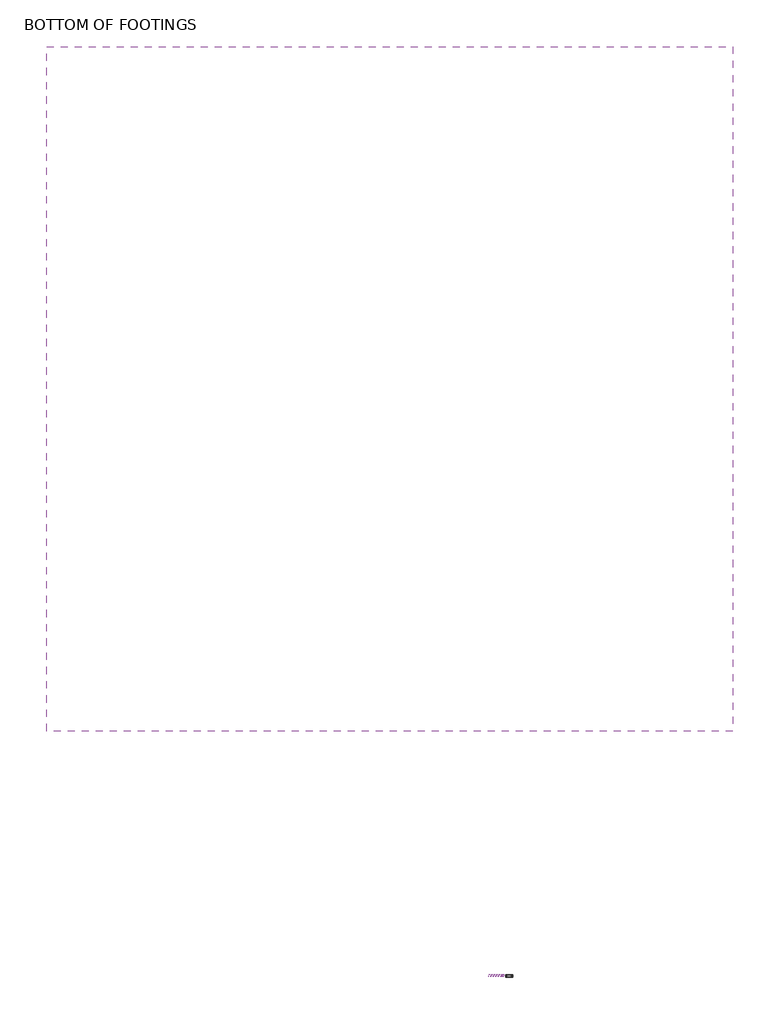
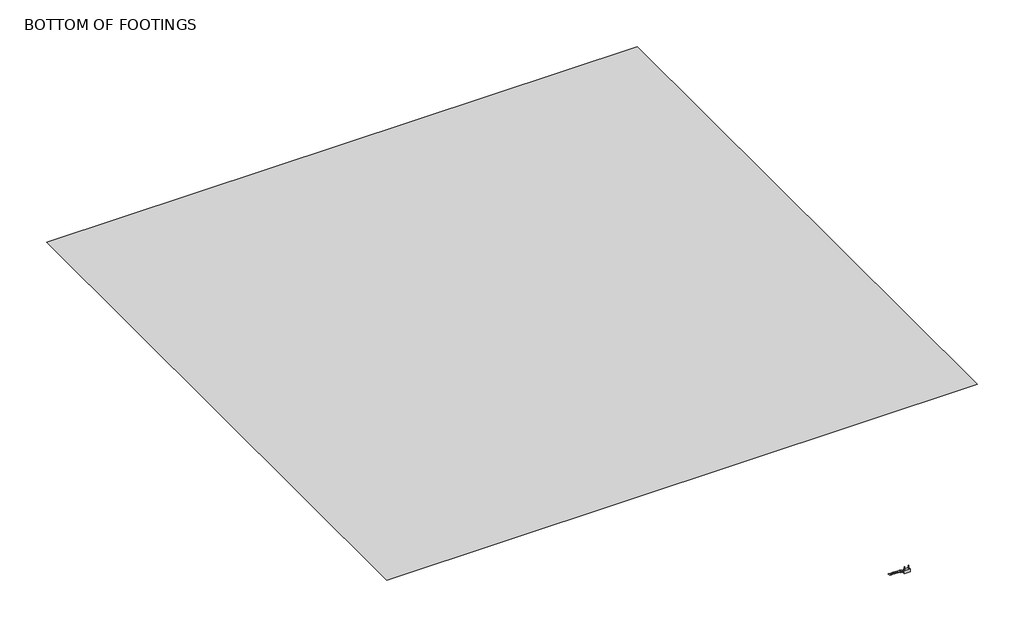
# One storey: 21 proxies.
"""IFC4 building model written with IfcOpenShell, lengths in millimetres."""

import ifcopenshell
import ifcopenshell.guid

model = None  # the IFC model being written
_history = None  # IfcOwnerHistory: only IFC2X3 demands one
_inside = {}  # id of a spatial element -> (the spatial element, [elements in it])
_under = {}  # id of a project, library or spatial element -> (it, [spatial elements below it])
_declared = {}  # id of a project -> (the project, [libraries it declares])
_typed = {}  # id of a type object -> (the type object, [elements of that type])
_made_of = {}  # id of a material, layer set ... -> (it, [elements and type objects made of it])


def new_model(schema):
    """Start an empty IFC model of exactly this schema.

    Asked for "IFC4X3", IfcOpenShell would pick the latest addendum, in which some entities
    have other attributes; the version numbers below select the first issue.
    IFC2X3 requires an IfcOwnerHistory on every rooted entity: one is made here for all.
    """
    global model, _history
    if schema == "IFC4X3":
        model = ifcopenshell.file(schema_version=(4, 3, 0, 0))
    else:
        model = ifcopenshell.file(schema=schema)
    _inside.clear()
    _under.clear()
    _declared.clear()
    _typed.clear()
    _made_of.clear()
    _history = None
    if model.schema == "IFC2X3":
        org = make("IfcOrganization", Name="unknown")
        user = make(
            "IfcPersonAndOrganization",
            ThePerson=make("IfcPerson", FamilyName="unknown"),
            TheOrganization=org,
        )
        app = make(
            "IfcApplication",
            ApplicationDeveloper=org,
            Version="unknown",
            ApplicationFullName="unknown",
            ApplicationIdentifier="unknown",
        )
        _history = make(
            "IfcOwnerHistory",
            OwningUser=user,
            OwningApplication=app,
            ChangeAction="ADDED",
            CreationDate=0,
        )
    return model


def make(cls, **values):
    """One entity of the class cls with the attributes given. An attribute that is None is left unset."""
    return model.create_entity(
        cls, **{name: value for name, value in values.items() if value is not None}
    )


def rooted(cls, **values):
    """An entity with a GlobalId (a new one), such as an element, a storey or a relation."""
    return make(cls, GlobalId=ifcopenshell.guid.new(), OwnerHistory=_history, **values)


def si_unit(unit_type, name, prefix=None):
    """IfcSIUnit, for example si_unit("LENGTHUNIT", "METRE", prefix="MILLI")."""
    return make("IfcSIUnit", UnitType=unit_type, Prefix=prefix, Name=name)


def assignment(units):
    """IfcUnitAssignment: the units of a project."""
    return None if units is None else make("IfcUnitAssignment", Units=units)


def point(xyz):
    """IfcCartesianPoint."""
    return None if xyz is None else make("IfcCartesianPoint", Coordinates=xyz)


def direction(xyz):
    """IfcDirection."""
    return None if xyz is None else make("IfcDirection", DirectionRatios=xyz)


def frame(location, z_axis=None, x_axis=None):
    """IfcAxis2Placement3D, a coordinate frame: its origin and axes. An axis left out is left unset."""
    return make(
        "IfcAxis2Placement3D",
        Location=point(location),
        Axis=direction(z_axis),
        RefDirection=direction(x_axis),
    )


def frame_2d(location, x_axis=None):
    """IfcAxis2Placement2D, a coordinate frame in the plane: its origin and x axis."""
    return make(
        "IfcAxis2Placement2D", Location=point(location), RefDirection=direction(x_axis)
    )


def origin():
    """The frame at (0, 0, 0) with its axes left unset."""
    return frame((0.0, 0.0, 0.0))


def place(relative_to, where):
    """IfcLocalPlacement: puts the frame where relative to a parent placement (None: the world)."""
    return make(
        "IfcLocalPlacement", PlacementRelTo=relative_to, RelativePlacement=where
    )


def context(
    kind, dimensions, precision=None, world=None, true_north=None, identifier=None
):
    """IfcGeometricRepresentationContext, for example the 3D "Model" context."""
    return make(
        "IfcGeometricRepresentationContext",
        ContextIdentifier=identifier,
        ContextType=kind,
        CoordinateSpaceDimension=dimensions,
        Precision=precision,
        WorldCoordinateSystem=world,
        TrueNorth=true_north,
    )


def project(units=None, contexts=None):
    """IfcProject with its units and contexts."""
    return rooted(
        "IfcProject",
        Name="project",
        RepresentationContexts=contexts,
        UnitsInContext=assignment(units),
    )


def spatial(cls, under=None, at=None, **own):
    """A site, building, storey or space (cls), placed at a placement, below another one or the project."""
    s = rooted(cls, ObjectPlacement=at, **own)
    if under is not None:
        _under.setdefault(under.id(), (under, []))[1].append(s)
    return s


def polyline(points):
    """IfcPolyline through the points."""
    return make("IfcPolyline", Points=[point(p) for p in points])


def point_list(points):
    """IfcCartesianPointList2D or 3D."""
    cls = (
        "IfcCartesianPointList2D" if len(points[0]) == 2 else "IfcCartesianPointList3D"
    )
    return make(cls, CoordList=points)


def circle_curve(where, radius):
    """IfcCircle in the frame where."""
    return make("IfcCircle", Position=where, Radius=radius)


def trimmed(basis, trim1, trim2, sense, master):
    """IfcTrimmedCurve: the piece of a basis curve between two trims."""
    return make(
        "IfcTrimmedCurve",
        BasisCurve=basis,
        Trim1=trim1,
        Trim2=trim2,
        SenseAgreement=sense,
        MasterRepresentation=master,
    )


def segment(curve, same_sense, transition):
    """IfcCompositeCurveSegment."""
    return make(
        "IfcCompositeCurveSegment",
        Transition=transition,
        SameSense=same_sense,
        ParentCurve=curve,
    )


def composite_curve(segments, self_intersect=None):
    """IfcCompositeCurve: segments joined end to end."""
    return make("IfcCompositeCurve", Segments=segments, SelfIntersect=self_intersect)


def outline(outer, holes=None, kind="AREA"):
    """IfcArbitraryClosedProfileDef: a profile drawn as a closed curve; with holes, ...WithVoids."""
    if holes is None:
        return make("IfcArbitraryClosedProfileDef", ProfileType=kind, OuterCurve=outer)
    return make(
        "IfcArbitraryProfileDefWithVoids",
        ProfileType=kind,
        OuterCurve=outer,
        InnerCurves=holes,
    )


def extrude(swept, where, along, depth):
    """IfcExtrudedAreaSolid: the profile swept, set in the frame where, extruded along a direction by depth."""
    return make(
        "IfcExtrudedAreaSolid",
        SweptArea=swept,
        Position=where,
        ExtrudedDirection=direction(along),
        Depth=depth,
    )


def faces_of(points, faces, orient=None, outer=None):
    """IfcFace entities. A face is a list of loops; a loop is a list of indices into points, from 0.

    orient and outer hold one flag for each loop. By default every Orientation is true, the
    first loop of a face is its IfcFaceOuterBound and the others are IfcFaceBound.
    """
    made = []
    for i, loops in enumerate(faces):
        bounds = []
        for j, loop in enumerate(loops):
            is_outer = j == 0 if outer is None else outer[i][j]
            bounds.append(
                make(
                    "IfcFaceOuterBound" if is_outer else "IfcFaceBound",
                    Bound=make("IfcPolyLoop", Polygon=[points[k] for k in loop]),
                    Orientation=True if orient is None else orient[i][j],
                )
            )
        made.append(make("IfcFace", Bounds=bounds))
    return made


def faceted_brep(points, faces, orient=None, outer=None, voids=None):
    """IfcFacetedBrep: a solid bounded by flat faces; with voids (closed shells), ...WithVoids."""
    shared = [point(p) for p in points]
    hull = make("IfcClosedShell", CfsFaces=faces_of(shared, faces, orient, outer))
    if voids is None:
        return make("IfcFacetedBrep", Outer=hull)
    return make(
        "IfcFacetedBrepWithVoids",
        Outer=hull,
        Voids=[
            make(cls, CfsFaces=faces_of(shared, fs, o, b)) for cls, fs, o, b in voids
        ],
    )


def triangles(points, corners, closed=None, point_numbers=None):
    """IfcTriangulatedFaceSet: each triangle names its three corners, points numbered from 1."""
    return make(
        "IfcTriangulatedFaceSet",
        Coordinates=point_list(points),
        Closed=closed,
        CoordIndex=corners,
        PnIndex=point_numbers,
    )


def shape(context_of_items, identifier, shape_type, items):
    """IfcShapeRepresentation: the items that make up one representation, for example the "Body"."""
    return make(
        "IfcShapeRepresentation",
        ContextOfItems=context_of_items,
        RepresentationIdentifier=identifier,
        RepresentationType=shape_type,
        Items=items,
    )


def source(mapping_origin, context_of_items, identifier, shape_type, items):
    """IfcRepresentationMap: a shape defined once, which mapped items show again and again."""
    return make(
        "IfcRepresentationMap",
        MappingOrigin=mapping_origin,
        MappedRepresentation=shape(context_of_items, identifier, shape_type, items),
    )


def transform(
    local_origin,
    x_axis=None,
    y_axis=None,
    z_axis=None,
    scale=None,
    scale2=None,
    scale3=None,
    uniform=True,
):
    """IfcCartesianTransformationOperator3D, or its non-uniform kind. x_axis, y_axis, z_axis: its Axis1, 2, 3."""
    if uniform:
        return make(
            "IfcCartesianTransformationOperator3D",
            Axis1=direction(x_axis),
            Axis2=direction(y_axis),
            LocalOrigin=point(local_origin),
            Scale=scale,
            Axis3=direction(z_axis),
        )
    return make(
        "IfcCartesianTransformationOperator3DnonUniform",
        Axis1=direction(x_axis),
        Axis2=direction(y_axis),
        LocalOrigin=point(local_origin),
        Scale=scale,
        Axis3=direction(z_axis),
        Scale2=scale2,
        Scale3=scale3,
    )


def mapped(mapping_source, mapping_target):
    """IfcMappedItem: shows the shape of a source again, moved by a transform."""
    return make(
        "IfcMappedItem", MappingSource=mapping_source, MappingTarget=mapping_target
    )


def made_of(thing, what):
    """Note that an element or type object is made of a material, layer set ...; save() writes the relation."""
    if what is not None:
        _made_of.setdefault(what.id(), (what, []))[1].append(thing)
    return thing


def element(
    cls,
    number,
    at=None,
    inside=None,
    cuts=None,
    type_object=None,
    material=None,
    context=None,
    identifier="Body",
    shape_type=None,
    held_by="IfcProductDefinitionShape",
    body=None,
    shapes=None,
    **own,
):
    """One element of the class cls, such as IfcWall. Its Tag is "e" and its number.

    at: its placement. inside: the storey or other place that contains it. cuts: it is an
    opening in that element (IfcRelVoidsElement). A single representation is given by context,
    identifier, shape_type and body (its items); several are given by shapes. held_by: the class
    of the entity that holds the representations. save() writes the other relations.
    """
    e = rooted(cls, Tag="e%d" % number, ObjectPlacement=at, **own)
    if body is not None:
        shapes = [shape(context, identifier, shape_type, body)]
    if shapes is not None:
        e.Representation = make(held_by, Representations=shapes)
    if inside is not None:
        _inside.setdefault(inside.id(), (inside, []))[1].append(e)
    if cuts is not None:
        rooted(
            "IfcRelVoidsElement", RelatingBuildingElement=cuts, RelatedOpeningElement=e
        )
    if type_object is not None:
        _typed.setdefault(type_object.id(), (type_object, []))[1].append(e)
    return made_of(e, material)


def aggregate(whole, parts):
    """IfcRelAggregates: a whole, such as a stair, and the parts it consists of."""
    return rooted("IfcRelAggregates", RelatingObject=whole, RelatedObjects=parts)


def save(model, path):
    """Write the relations noted so far, then the file.

    IfcRelAggregates (storeys below a building ...), IfcRelContainedInSpatialStructure (elements
    in a storey), IfcRelDefinesByType, IfcRelAssociatesMaterial and IfcRelDeclares: one each for
    every whole, place, type object, material and project.
    """
    for whole, parts in _under.values():
        aggregate(whole, parts)
    for where, things in _inside.values():
        rooted(
            "IfcRelContainedInSpatialStructure",
            RelatedElements=things,
            RelatingStructure=where,
        )
    for kind, things in _typed.values():
        rooted("IfcRelDefinesByType", RelatedObjects=things, RelatingType=kind)
    for what, things in _made_of.values():
        rooted("IfcRelAssociatesMaterial", RelatedObjects=things, RelatingMaterial=what)
    for by, libraries in _declared.values():
        rooted("IfcRelDeclares", RelatingContext=by, RelatedDefinitions=libraries)
    model.write(path)


def plane_surface(at):
    """IfcPlane: the flat surface through the origin of the frame at, square to its z axis."""
    return make("IfcPlane", Position=at)


def revolved_surface(curve, axis_point, axis_direction):
    """IfcSurfaceOfRevolution: the curve turned about the line through axis_point along axis_direction."""
    return make(
        "IfcSurfaceOfRevolution",
        SweptCurve=make("IfcArbitraryOpenProfileDef", ProfileType="CURVE", Curve=curve),
        AxisPosition=make("IfcAxis1Placement", Location=point(axis_point), Axis=direction(axis_direction)),
    )


def advanced_brep(points, edges, surfaces, faces):
    """IfcAdvancedBrep: a solid bounded by faces that lie on surfaces and meet in shared edges.

    An edge is (start, end): straight between two places in points (the first is 0);
    or (start, end, curve); or (start, end, curve, False) where it runs against its curve.
    A face is (place in surfaces, loops), or (place, loops, False) where it looks against
    its surface's normal. A loop lists edges by number (the first is 1), with a minus sign
    where the edge is run from its end to its start. The first loop is the outer one.
    """
    corners = [point(p) for p in points]
    vertices = [make("IfcVertexPoint", VertexGeometry=c) for c in corners]
    made = []
    for start, end, *more in edges:
        made.append(
            make(
                "IfcEdgeCurve",
                EdgeStart=vertices[start],
                EdgeEnd=vertices[end],
                EdgeGeometry=more[0] if more else make("IfcPolyline", Points=[corners[start], corners[end]]),
                SameSense=more[1] if len(more) > 1 else True,
            )
        )
    hull = []
    for where, loops, *sense in faces:
        bounds = []
        for j, loop in enumerate(loops):
            ring = [make("IfcOrientedEdge", EdgeElement=made[abs(k) - 1], Orientation=k > 0) for k in loop]
            bounds.append(
                make(
                    "IfcFaceOuterBound" if j == 0 else "IfcFaceBound",
                    Bound=make("IfcEdgeLoop", EdgeList=ring),
                    Orientation=True,
                )
            )
        hull.append(make("IfcAdvancedFace", Bounds=bounds, FaceSurface=surfaces[where], SameSense=sense[0] if sense else True))
    return make("IfcAdvancedBrep", Outer=make("IfcClosedShell", CfsFaces=hull))


def generic_models_129_generic_models_1_8999e842(model_context):
    return source(origin(), model_context, "Body", "SweptSolid", [
        extrude(outline(polyline([(47499.4360531, 0.0), (46280.2360531, 0.0), (46280.2360531, 1219.2), (47499.4360531, 1219.2), (47499.4360531, 0.0)])), frame((0.0, 0.0, -378.376067), z_axis=(0.0, 0.0, 1.0), x_axis=(1.0, 0.0, 0.0)), (0.0, 0.0, 1.0), 152.4),
    ])


def generic_models_131_generic_models_1_dfd9233a(model_context):
    return source(origin(), model_context, "Body", "SweptSolid", [
        extrude(outline(polyline([(-223.594817, 46885.2894531), (-224.388567, 46885.2894531), (-224.388567, 46887.8393167), (-275.188567, 46889.4367058), (-275.188567, 46890.2354003), (-224.388567, 46891.8327895), (-224.388567, 46894.3826531), (-223.594817, 46894.3826531), (-223.594817, 46885.2894531)])), frame((0.0, 565.15, 0.0), z_axis=(0.0, 1.0, 0.0), x_axis=(0.0, 0.0, 1.0)), (0.0, 0.0, 1.0), 12.7),
    ])


def generic_models_139_generic_models_1_e596f594(model_context):
    return source(origin(), model_context, "Body", "SweptSolid", [
        extrude(outline(composite_curve([segment(trimmed(circle_curve(frame_2d((97.5288266, 52112.9548165)), 6.35), [point((91.1788266, 52112.9548165))], [point((103.8788266, 52112.9548165))], False, "CARTESIAN"), True, "CONTINUOUS"), segment(trimmed(circle_curve(frame_2d((97.5288266, 52112.9548165)), 6.35), [point((103.8788266, 52112.9548165))], [point((91.1788266, 52112.9548165))], False, "CARTESIAN"), True, "CONTINUOUS")], self_intersect=False)), frame((0.0, 0.0, 0.0), z_axis=(0.0, 1.0, 0.0), x_axis=(0.0, 0.0, 1.0)), (0.0, 0.0, 1.0), 1219.2),
    ])


def generic_models_141_generic_models_1_a1e14504(model_context):
    return source(origin(), model_context, "Body", "SweptSolid", [
        extrude(outline(composite_curve([segment(trimmed(circle_curve(frame_2d((-554.7288266, 52112.9548165)), 6.35), [point((-548.3788266, 52112.9548165))], [point((-561.0788266, 52112.9548165))], False, "CARTESIAN"), True, "CONTINUOUS"), segment(trimmed(circle_curve(frame_2d((-554.7288266, 52112.9548165)), 6.35), [point((-561.0788266, 52112.9548165))], [point((-548.3788266, 52112.9548165))], False, "CARTESIAN"), True, "CONTINUOUS")], self_intersect=False)), frame((0.0, 0.0, 0.0), z_axis=(0.0, 1.0, 0.0), x_axis=(0.0, 0.0, 1.0)), (0.0, 0.0, 1.0), 1219.2),
    ])


def generic_models_144_generic_models_1_4ebe4832(model_context):
    return source(origin(), model_context, "Body", "SweptSolid", [
        extrude(outline(polyline([(-79.375, 52785.9625), (-73.025, 52785.9625), (-73.025, 52209.6280698), (-272.1843039, 52010.4687659), (-276.674432, 52014.9588939), (-79.375, 52212.2583259), (-79.375, 52785.9625)])), frame((0.0, 0.0, 0.0), z_axis=(0.0, 1.0, 0.0), x_axis=(0.0, 0.0, 1.0)), (0.0, 0.0, 1.0), 1219.2),
    ])


def generic_models_145_generic_models_1_d1ee8326(model_context):
    return source(origin(), model_context, "Body", "SweptSolid", [
        extrude(outline(polyline([(-155.575, 52785.9625), (-153.9875, 52785.9625), (-153.9875, 52482.353125), (-458.7875, 52177.553125), (-458.7875, 51873.410689), (-460.375, 51873.410689), (-460.375, 52178.210689), (-155.575, 52483.010689), (-155.575, 52785.9625)])), frame((0.0, 0.0, 0.0), z_axis=(0.0, 1.0, 0.0), x_axis=(0.0, 0.0, 1.0)), (0.0, 0.0, 1.0), 1219.2),
    ])


def generic_models_150_generic_models_1_b2c8ea2b(model_context):
    return source(origin(), model_context, "Body", "SweptSolid", [
        extrude(outline(polyline([(-310.1710164, 52787.3395874), (-157.7710164, 52787.3395874), (-157.7710164, 52483.7302124), (-462.5710164, 52178.9302124), (-462.5710164, 51824.8420742), (-513.3710164, 51824.8420742), (-513.3710164, 52343.6563593), (-310.1710164, 52546.8563593), (-310.1710164, 52787.3395874)])), frame((0.0, 0.0, 0.0), z_axis=(0.0, 1.0, 0.0), x_axis=(0.0, 0.0, 1.0)), (0.0, 0.0, 1.0), 1219.2),
    ])


def generic_models_151_generic_models_1_08f1ca75(model_context):
    return source(origin(), model_context, "Body", "SweptSolid", [
        extrude(outline(polyline([(-76.2, 51566.7625), (-685.8, 51566.7625), (-685.8, 52787.3395874), (-310.1710164, 52787.3395874), (-310.1710164, 52546.8563593), (-513.3710164, 52343.6563593), (-513.3710164, 51824.8420742), (-462.5710164, 51824.8420742), (-462.5710164, 51871.5625), (-47.9216734, 51871.5625), (-76.2, 51566.7625)])), frame((0.0, 0.0, 0.0), z_axis=(0.0, 1.0, 0.0), x_axis=(0.0, 0.0, 1.0)), (0.0, 0.0, 1.0), 1219.2),
    ])


def generic_models_177_generic_models_1_1d143019(model_context):
    return source(origin(), model_context, "Body", "Brep", [
        faceted_brep([(56665.8125, 528.6375, -1066.8), (56526.1125, 528.6375, -1066.8), (56526.1125, 528.6375, 1809.75), (56665.8125, 528.6375, 1809.75), (56665.8125, 388.9375, -1066.8), (56665.8125, 388.9375, 1809.75), (56526.1125, 388.9375, 1809.75), (56526.1125, 388.9375, -1066.8), (56545.1625, 407.9875, 1828.8), (56646.7625, 407.9875, 1828.8), (56646.7625, 509.5875, 1828.8), (56545.1625, 509.5875, 1828.8)], [[[0, 1, 2, 3]], [[4, 5, 6, 7]], [[1, 0, 4, 7]], [[2, 1, 7, 6]], [[8, 9, 10, 11]], [[0, 3, 5, 4]], [[2, 6, 8, 11]], [[5, 3, 10, 9]], [[6, 5, 9, 8]], [[3, 2, 11, 10]]]),
    ])


def generic_models_178_generic_models_155_a54ccf4c(model_context):
    return source(origin(), model_context, "Body", "SweptSolid", [
        extrude(outline(composite_curve([segment(trimmed(circle_curve(frame_2d((56595.9625, 458.7875)), 152.4), [point((56443.5625, 458.7875))], [point((56748.3625, 458.7875))], False, "CARTESIAN"), True, "CONTINUOUS"), segment(trimmed(circle_curve(frame_2d((56595.9625, 458.7875)), 152.4), [point((56748.3625, 458.7875))], [point((56443.5625, 458.7875))], False, "CARTESIAN"), True, "CONTINUOUS")], self_intersect=False)), frame((0.0, 0.0, -1219.2), z_axis=(0.0, 0.0, 1.0), x_axis=(1.0, 0.0, 0.0)), (0.0, 0.0, 1.0), 1219.2),
        extrude(outline(composite_curve([segment(trimmed(circle_curve(frame_2d((54157.5625, 458.7875)), 152.4), [point((54005.1625, 458.7875))], [point((54309.9625, 458.7875))], False, "CARTESIAN"), True, "CONTINUOUS"), segment(trimmed(circle_curve(frame_2d((54157.5625, 458.7875)), 152.4), [point((54309.9625, 458.7875))], [point((54005.1625, 458.7875))], False, "CARTESIAN"), True, "CONTINUOUS")], self_intersect=False)), frame((0.0, 0.0, -1219.2), z_axis=(0.0, 0.0, 1.0), x_axis=(1.0, 0.0, 0.0)), (0.0, 0.0, 1.0), 1219.2),
    ])


def generic_models_183_generic_models_1_4255d89c(model_context):
    return source(origin(), model_context, "Body", "Brep", [
        faceted_brep([(54227.4125, 528.6375, -1066.8), (54087.7125, 528.6375, -1066.8), (54087.7125, 528.6375, 1809.75), (54227.4125, 528.6375, 1809.75), (54227.4125, 388.9375, -1066.8), (54227.4125, 388.9375, 1809.75), (54087.7125, 388.9375, 1809.75), (54087.7125, 388.9375, -1066.8), (54106.7625, 407.9875, 1828.8), (54208.3625, 407.9875, 1828.8), (54208.3625, 509.5875, 1828.8), (54106.7625, 509.5875, 1828.8)], [[[0, 1, 2, 3]], [[4, 5, 6, 7]], [[1, 0, 4, 7]], [[2, 1, 7, 6]], [[8, 9, 10, 11]], [[0, 3, 5, 4]], [[2, 6, 8, 11]], [[5, 3, 10, 9]], [[6, 5, 9, 8]], [[3, 2, 11, 10]]]),
    ])


def generic_models_184_generic_models_184_067f22a4(model_context):
    return source(origin(), model_context, "Body", "AdvancedBrep", [
        advanced_brep(
        [(57021.4125, 977.9, -23.9117188), (53732.1125, 977.9, -23.9117188), (53732.1125, -241.3, -23.9117188), (57021.4125, -241.3, -23.9117188), (56443.5625, 458.7875, -23.9117188), (56748.3625, 458.7875, -23.9117188), (54005.1625, 458.7875, -23.9117188), (54309.9625, 458.7875, -23.9117188), (57021.4125, 977.9, -1915.3720904), (57021.4125, -241.3, -1915.3720904), (53732.1125, -241.3, -1915.3720904), (53732.1125, 977.9, -1915.3720904), (56443.5625, 458.7875, -1219.2), (56748.3625, 458.7875, -1219.2), (54005.1625, 458.7875, -1219.2), (54309.9625, 458.7875, -1219.2)],
        [
            (0, 1),
            (1, 2),
            (2, 3),
            (3, 0),
            (4, 5, circle_curve(frame((56595.9625, 458.7875, -23.9117188), z_axis=(0.0, 0.0, -1.0), x_axis=(1.0, 0.0, 0.0)), 152.4)),
            (5, 4, circle_curve(frame((56595.9625, 458.7875, -23.9117188), z_axis=(0.0, 0.0, -1.0), x_axis=(1.0, 0.0, 0.0)), 152.4)),
            (6, 7, circle_curve(frame((54157.5625, 458.7875, -23.9117188), z_axis=(0.0, 0.0, -1.0), x_axis=(1.0, 0.0, 0.0)), 152.4)),
            (7, 6, circle_curve(frame((54157.5625, 458.7875, -23.9117188), z_axis=(0.0, 0.0, -1.0), x_axis=(1.0, 0.0, 0.0)), 152.4)),
            (8, 9),
            (9, 10),
            (10, 11),
            (11, 8),
            (0, 8),
            (11, 1),
            (10, 2),
            (9, 3),
            (12, 13, circle_curve(frame((56595.9625, 458.7875, -1219.2), z_axis=(0.0, 0.0, 1.0), x_axis=(1.0, 0.0, 0.0)), 152.4)),
            (13, 12, circle_curve(frame((56595.9625, 458.7875, -1219.2), z_axis=(0.0, 0.0, 1.0), x_axis=(1.0, 0.0, 0.0)), 152.4)),
            (14, 15, circle_curve(frame((54157.5625, 458.7875, -1219.2), z_axis=(0.0, 0.0, 1.0), x_axis=(1.0, 0.0, 0.0)), 152.4)),
            (15, 14, circle_curve(frame((54157.5625, 458.7875, -1219.2), z_axis=(0.0, 0.0, 1.0), x_axis=(1.0, 0.0, 0.0)), 152.4)),
            (13, 5),
            (4, 12),
            (15, 7),
            (6, 14),
        ],
        [
            plane_surface(frame((53732.1125, 977.9, -23.9117188), z_axis=(0.0, 0.0, 1.0), x_axis=(-1.0, 0.0, 0.0))),
            plane_surface(frame((53732.1125, 977.9, -1915.3720904), z_axis=(0.0, 0.0, -1.0), x_axis=(1.0, 0.0, 0.0))),
            plane_surface(frame((57021.4125, 977.9, -23.9117188), z_axis=(0.0, 1.0, 0.0), x_axis=(0.0, 0.0, -1.0))),
            plane_surface(frame((53732.1125, 977.9, -23.9117188), z_axis=(-1.0, 0.0, 0.0), x_axis=(0.0, 0.0, -1.0))),
            plane_surface(frame((53732.1125, -241.3, -23.9117188), z_axis=(0.0, -1.0, 0.0), x_axis=(0.0, 0.0, -1.0))),
            plane_surface(frame((57021.4125, -241.3, -23.9117188), z_axis=(1.0, 0.0, 0.0), x_axis=(0.0, 0.0, -1.0))),
            plane_surface(frame((56748.3625, 458.7875, -1219.2), z_axis=(0.0, 0.0, 1.0), x_axis=(0.0, -1.0, 0.0))),
            revolved_surface(polyline([(56748.3625, 458.7875, -23.911718800000017), (56748.3625, 458.7875, -1219.2)]), (56595.9625, 458.7875, -1219.2), (0.0, 0.0, 1.0)),
            revolved_surface(polyline([(54309.9625, 458.7875, -23.9117188), (54309.9625, 458.7875, -1219.2)]), (54157.5625, 458.7875, 0.0), (0.0, 0.0, 1.0)),
        ],
        [
            (0, [[1, 2, 3, 4], [5, 6], [7, 8]]),
            (1, [[9, 10, 11, 12]]),
            (2, [[-1, 13, -12, 14]]),
            (3, [[-2, -14, -11, 15]]),
            (4, [[-3, -15, -10, 16]]),
            (5, [[-4, -16, -9, -13]]),
            (6, [[17, 18]]),
            (6, [[19, 20]]),
            (7, [[-18, 21, -5, 22]]),
            (7, [[-17, -22, -6, -21]]),
            (8, [[-20, 23, -7, 24]]),
            (8, [[-19, -24, -8, -23]]),
        ],
    ),
    ])


def generic_models_11_generic_models_1_850b304e(model_context):
    return source(origin(), model_context, "Body", "SweptSolid", [
        extrude(outline(polyline([(50347.5625, 0.0), (49128.3625, 0.0), (49128.3625, 1219.2), (50347.5625, 1219.2), (50347.5625, 0.0)])), frame((0.0, 0.0, -152.4), z_axis=(0.0, 0.0, 1.0), x_axis=(1.0, 0.0, 0.0)), (0.0, 0.0, 1.0), 152.4),
    ])


def generic_models_201_generic_models_1_6cd63f98(model_context):
    return source(origin(), model_context, "Body", "SweptSolid", [
        extrude(outline(polyline([(2.38125, 49733.4159), (1.5875, 49733.4159), (1.5875, 49735.9657636), (-49.2125, 49737.5631527), (-49.2125, 49738.3618473), (1.5875, 49739.9592364), (1.5875, 49742.5091), (2.38125, 49742.5091), (2.38125, 49733.4159)])), frame((0.0, 565.15, 0.0), z_axis=(0.0, 1.0, 0.0), x_axis=(0.0, 0.0, 1.0)), (0.0, 0.0, 1.0), 12.7),
    ])


def generic_models_8_generic_models_1_dd7fddfd(model_context):
    return source(origin(), model_context, "Body", "SweptSolid", [
        extrude(outline(polyline([(0.0, 52785.9625), (0.0, 51871.5625), (-457.2, 51871.5625), (-457.2, 52176.3625), (-152.4, 52481.1625), (-152.4, 52785.9625), (-79.375, 52785.9625), (-79.375, 52212.2583259), (-276.674432, 52014.9588939), (-272.1843039, 52010.4687659), (-73.025, 52209.6280698), (-73.025, 52785.9625), (0.0, 52785.9625)]), holes=[composite_curve([segment(trimmed(circle_curve(frame_2d((-76.2, 51947.7625)), 6.35), [point((-69.85, 51947.7625))], [point((-82.55, 51947.7625))], True, "CARTESIAN"), True, "CONTINUOUS"), segment(trimmed(circle_curve(frame_2d((-76.2, 51947.7625)), 6.35), [point((-82.55, 51947.7625))], [point((-69.85, 51947.7625))], True, "CARTESIAN"), True, "CONTINUOUS")], self_intersect=False), composite_curve([segment(trimmed(circle_curve(frame_2d((-381.0, 51947.7625)), 6.35), [point((-374.65, 51947.7625))], [point((-387.35, 51947.7625))], True, "CARTESIAN"), True, "CONTINUOUS"), segment(trimmed(circle_curve(frame_2d((-381.0, 51947.7625)), 6.35), [point((-387.35, 51947.7625))], [point((-374.65, 51947.7625))], True, "CARTESIAN"), True, "CONTINUOUS")], self_intersect=False)]), frame((0.0, 0.0, 0.0), z_axis=(0.0, 1.0, 0.0), x_axis=(0.0, 0.0, 1.0)), (0.0, 0.0, 1.0), 1219.2),
    ])


model = new_model("IFC4")

# Units and contexts
model_context = context("Model", 3, world=origin())
ifc_project = project(units=[si_unit("LENGTHUNIT", "METRE", prefix="MILLI")], contexts=[model_context])

# Site, building, storey
site = spatial("IfcSite", under=ifc_project)
building = spatial("IfcBuilding", under=site)
storey = spatial("IfcBuildingStorey", under=building, Name="BOTTOM OF FOOTINGS", Elevation=-2032.0)

# Proxies
placement = place(None, origin())
element("IfcBuildingElementProxy", 1, Name="Building Element Proxy", at=placement, inside=storey, context=model_context, shape_type="Tessellation", body=[
    triangles([(-171822.2005371, 120741.2254395, -152.4), (165286.5994629, 120741.2254395, -152.4), (165286.5994629, 456935.644043, -152.4), (-171822.2005371, 456935.644043, -152.4)], [[4, 1, 2], [2, 3, 4]], closed=False),
])
generic_models_129_generic_models_1_shape = generic_models_129_generic_models_1_8999e842(model_context)
element("IfcBuildingElementProxy", 2, Name="Generic Models 129 : Generic Models 1", ObjectType="Generic Models 129 : Generic Models 1", at=placement, inside=storey, context=model_context, shape_type="MappedRepresentation", body=[
    mapped(generic_models_129_generic_models_1_shape, transform((4067.3264469, 0.0, 225.976067), x_axis=(1.0, 0.0, 0.0), y_axis=(0.0, 1.0, 0.0), z_axis=(0.0, 0.0, 1.0))),
])
generic_models_131_generic_models_1_shape = generic_models_131_generic_models_1_dfd9233a(model_context)
element("IfcBuildingElementProxy", 3, Name="Generic Models 131 : Generic Models 1", ObjectType="Generic Models 131 : Generic Models 1", at=placement, inside=storey, context=model_context, shape_type="MappedRepresentation", body=[
    mapped(generic_models_131_generic_models_1_shape, transform((1628.9264469, 0.0, 225.976067), x_axis=(1.0, 0.0, 0.0), y_axis=(0.0, 1.0, 0.0), z_axis=(0.0, 0.0, 1.0))),
])
generic_models_139_generic_models_1_shape = generic_models_139_generic_models_1_e596f594(model_context)
element("IfcBuildingElementProxy", 4, Name="Generic Models 139 : Generic Models 1", ObjectType="Generic Models 139 : Generic Models 1", at=placement, inside=storey, context=model_context, shape_type="MappedRepresentation", body=[
    mapped(generic_models_139_generic_models_1_shape, transform((-165.1923165, 0.0, -173.7288266), x_axis=(1.0, 0.0, 0.0), y_axis=(0.0, 1.0, 0.0), z_axis=(0.0, 0.0, 1.0))),
])
generic_models_141_generic_models_1_shape = generic_models_141_generic_models_1_a1e14504(model_context)
element("IfcBuildingElementProxy", 5, Name="Generic Models 141 : Generic Models 1", ObjectType="Generic Models 141 : Generic Models 1", at=placement, inside=storey, context=model_context, shape_type="MappedRepresentation", body=[
    mapped(generic_models_141_generic_models_1_shape, transform((-165.1923165, 0.0, 173.7288266), x_axis=(1.0, 0.0, 0.0), y_axis=(0.0, 1.0, 0.0), z_axis=(0.0, 0.0, 1.0))),
])
generic_models_144_generic_models_1_shape = generic_models_144_generic_models_1_4ebe4832(model_context)
element("IfcBuildingElementProxy", 6, Name="Generic Models 144 : Generic Models 1", ObjectType="Generic Models 144 : Generic Models 1", at=placement, inside=storey, context=model_context, shape_type="MappedRepresentation", body=[
    mapped(generic_models_144_generic_models_1_shape, transform((0.0, 0.0, 0.0), x_axis=(1.0, 0.0, 0.0), y_axis=(0.0, 1.0, 0.0), z_axis=(0.0, 0.0, 1.0))),
])
generic_models_145_generic_models_1_shape = generic_models_145_generic_models_1_d1ee8326(model_context)
element("IfcBuildingElementProxy", 7, Name="Generic Models 145 : Generic Models 1", ObjectType="Generic Models 145 : Generic Models 1", at=placement, inside=storey, context=model_context, shape_type="MappedRepresentation", body=[
    mapped(generic_models_145_generic_models_1_shape, transform((0.0, 0.0, 0.0), x_axis=(1.0, 0.0, 0.0), y_axis=(0.0, 1.0, 0.0), z_axis=(0.0, 0.0, 1.0))),
])
generic_models_150_generic_models_1_shape = generic_models_150_generic_models_1_b2c8ea2b(model_context)
element("IfcBuildingElementProxy", 8, Name="Generic Models 150 : Generic Models 1", ObjectType="Generic Models 150 : Generic Models 1", at=placement, inside=storey, context=model_context, shape_type="MappedRepresentation", body=[
    mapped(generic_models_150_generic_models_1_shape, transform((0.0, 0.0, 0.0), x_axis=(1.0, 0.0, 0.0), y_axis=(0.0, 1.0, 0.0), z_axis=(0.0, 0.0, 1.0))),
])
generic_models_151_generic_models_1_shape = generic_models_151_generic_models_1_08f1ca75(model_context)
element("IfcBuildingElementProxy", 9, Name="Generic Models 151 : Generic Models 1", ObjectType="Generic Models 151 : Generic Models 1", at=placement, inside=storey, context=model_context, shape_type="MappedRepresentation", body=[
    mapped(generic_models_151_generic_models_1_shape, transform((0.0, 0.0, 0.0), x_axis=(1.0, 0.0, 0.0), y_axis=(0.0, 1.0, 0.0), z_axis=(0.0, 0.0, 1.0))),
])
generic_models_177_generic_models_1_shape = generic_models_177_generic_models_1_1d143019(model_context)
element("IfcBuildingElementProxy", 10, Name="Generic Models 177 : Generic Models 1", ObjectType="Generic Models 177 : Generic Models 1", at=placement, inside=storey, context=model_context, shape_type="MappedRepresentation", body=[
    mapped(generic_models_177_generic_models_1_shape, transform((0.0, 0.0, 0.0), x_axis=(1.0, 0.0, 0.0), y_axis=(0.0, 1.0, 0.0), z_axis=(0.0, 0.0, 1.0))),
])
generic_models_178_generic_models_155_shape = generic_models_178_generic_models_155_a54ccf4c(model_context)
element("IfcBuildingElementProxy", 11, Name="Generic Models 178 : Generic Models 155", ObjectType="Generic Models 178 : Generic Models 155", at=placement, inside=storey, context=model_context, shape_type="MappedRepresentation", body=[
    mapped(generic_models_178_generic_models_155_shape, transform((0.0, 0.0, 0.0), x_axis=(1.0, 0.0, 0.0), y_axis=(0.0, 1.0, 0.0), z_axis=(0.0, 0.0, 1.0))),
])
generic_models_183_generic_models_1_shape = generic_models_183_generic_models_1_4255d89c(model_context)
element("IfcBuildingElementProxy", 12, Name="Generic Models 183 : Generic Models 1", ObjectType="Generic Models 183 : Generic Models 1", at=placement, inside=storey, context=model_context, shape_type="MappedRepresentation", body=[
    mapped(generic_models_183_generic_models_1_shape, transform((0.0, 0.0, 0.0), x_axis=(1.0, 0.0, 0.0), y_axis=(0.0, 1.0, 0.0), z_axis=(0.0, 0.0, 1.0))),
])
generic_models_184_generic_models_184_shape = generic_models_184_generic_models_184_067f22a4(model_context)
element("IfcBuildingElementProxy", 13, Name="Generic Models 184 : Generic Models 184", ObjectType="Generic Models 184 : Generic Models 184", at=placement, inside=storey, context=model_context, shape_type="MappedRepresentation", body=[
    mapped(generic_models_184_generic_models_184_shape, transform((0.0, 0.0, 0.0), x_axis=(1.0, 0.0, 0.0), y_axis=(0.0, 1.0, 0.0), z_axis=(0.0, 0.0, 1.0))),
])
generic_models_11_generic_models_1_shape = generic_models_11_generic_models_1_850b304e(model_context)
element("IfcBuildingElementProxy", 14, Name="Generic Models 190 : Generic Models 1", ObjectType="Generic Models 190 : Generic Models 1", at=placement, inside=storey, context=model_context, shape_type="MappedRepresentation", body=[
    mapped(generic_models_11_generic_models_1_shape, transform((-2438.4, 0.0, 0.0), x_axis=(1.0, 0.0, 0.0), y_axis=(0.0, 1.0, 0.0), z_axis=(0.0, 0.0, 1.0))),
])
generic_models_201_generic_models_1_shape = generic_models_201_generic_models_1_6cd63f98(model_context)
element("IfcBuildingElementProxy", 15, Name="Generic Models 201 : Generic Models 1", ObjectType="Generic Models 201 : Generic Models 1", at=placement, inside=storey, context=model_context, shape_type="MappedRepresentation", body=[
    mapped(generic_models_201_generic_models_1_shape, transform((-2438.4, 0.0, 0.0), x_axis=(1.0, 0.0, 0.0), y_axis=(0.0, 1.0, 0.0), z_axis=(0.0, 0.0, 1.0))),
])
element("IfcBuildingElementProxy", 16, Name="Generic Models 210 : Generic Models 1", ObjectType="Generic Models 210 : Generic Models 1", at=placement, inside=storey, context=model_context, shape_type="MappedRepresentation", body=[
    mapped(generic_models_11_generic_models_1_shape, transform((-3657.6, 0.0, 0.0), x_axis=(1.0, 0.0, 0.0), y_axis=(0.0, 1.0, 0.0), z_axis=(0.0, 0.0, 1.0))),
])
element("IfcBuildingElementProxy", 17, Name="Generic Models 218 : Generic Models 1", ObjectType="Generic Models 218 : Generic Models 1", at=placement, inside=storey, context=model_context, shape_type="MappedRepresentation", body=[
    mapped(generic_models_201_generic_models_1_shape, transform((-3657.6, 0.0, 0.0), x_axis=(1.0, 0.0, 0.0), y_axis=(0.0, 1.0, 0.0), z_axis=(0.0, 0.0, 1.0))),
])
element("IfcBuildingElementProxy", 18, Name="Generic Models 28 : Generic Models 1", ObjectType="Generic Models 28 : Generic Models 1", at=placement, inside=storey, context=model_context, shape_type="MappedRepresentation", body=[
    mapped(generic_models_11_generic_models_1_shape, transform((0.0, 0.0, 0.0), x_axis=(1.0, 0.0, 0.0), y_axis=(0.0, 1.0, 0.0), z_axis=(0.0, 0.0, 1.0))),
])
element("IfcBuildingElementProxy", 19, Name="Generic Models 38 : Generic Models 1", ObjectType="Generic Models 38 : Generic Models 1", at=placement, inside=storey, context=model_context, shape_type="MappedRepresentation", body=[
    mapped(generic_models_201_generic_models_1_shape, transform((0.0, 0.0, 0.0), x_axis=(1.0, 0.0, 0.0), y_axis=(0.0, 1.0, 0.0), z_axis=(0.0, 0.0, 1.0))),
])
generic_models_8_generic_models_1_shape = generic_models_8_generic_models_1_dd7fddfd(model_context)
element("IfcBuildingElementProxy", 20, Name="Generic Models 8 : Generic Models 1", ObjectType="Generic Models 8 : Generic Models 1", at=placement, inside=storey, context=model_context, shape_type="MappedRepresentation", body=[
    mapped(generic_models_8_generic_models_1_shape, transform((0.0, 0.0, 0.0), x_axis=(1.0, 0.0, 0.0), y_axis=(0.0, 1.0, 0.0), z_axis=(0.0, 0.0, 1.0))),
])
element("IfcBuildingElementProxy", 21, Name="Generic Models 96 : Generic Models 1", ObjectType="Generic Models 96 : Generic Models 1", at=placement, inside=storey, context=model_context, shape_type="MappedRepresentation", body=[
    mapped(generic_models_129_generic_models_1_shape, transform((1628.9264469, 0.0, 225.976067), x_axis=(1.0, 0.0, 0.0), y_axis=(0.0, 1.0, 0.0), z_axis=(0.0, 0.0, 1.0))),
])

save(model, "model.ifc")

# Revit data of these elements
# Project information
#   Project Issue Date = "06/12/2018"
#   Project Status = "Project Status"
#   Client Name = "Owner"
#   Project Address = "5253 KING JAMES WAY, FITCHBURG, WI"
#   Project Name = "FORAGE KOMBUCHA"
#   Project Number = "Project Number"
# Element 1 (IfcBuildingElementProxy)
#   Material = none
#   Phase Created = 1st Phase
# Element 2 (IfcBuildingElementProxy, "Generic Models 129 : Generic Models 1")
#   Phase Created = _SAVE
#   Materials on its faces: "EXISTING SLAB"
# Element 3 (IfcBuildingElementProxy, "Generic Models 131 : Generic Models 1")
#   Phase Created = _SAVE
#   Materials on its faces: "METAL RUNNER CHANNEL; FASTEN @ 24\" O.C."
# Element 4 (IfcBuildingElementProxy, "Generic Models 139 : Generic Models 1")
#   Phase Created = _SAVE
#   Materials on its faces: "#4 CONT. STEEL REBAR"
# Element 5 (IfcBuildingElementProxy, "Generic Models 141 : Generic Models 1")
#   Phase Created = _SAVE
#   Materials on its faces: "#4 CONT. STEEL REBAR"
# Element 6 (IfcBuildingElementProxy, "Generic Models 144 : Generic Models 1")
#   Phase Created = _SAVE
#   Materials on its faces: "#10 6x6 WIRE MESH"
# Element 7 (IfcBuildingElementProxy, "Generic Models 145 : Generic Models 1")
#   Phase Created = _SAVE
#   Materials on its faces: "6 MIL VAPOR BARRIER"
# Element 8 (IfcBuildingElementProxy, "Generic Models 150 : Generic Models 1")
#   Phase Created = _SAVE
#   Materials on its faces: "6\" COMPACTED CRUSHED STONE"
# Element 9 (IfcBuildingElementProxy, "Generic Models 151 : Generic Models 1")
#   Phase Created = _SAVE
#   Materials on its faces: "GRADE (SLOPE 2% MIN AWAY FROM BUILDING)"
# Element 10 (IfcBuildingElementProxy, "Generic Models 177 : Generic Models 1")
#   Phase Created = _SAVE
#   Materials on its faces: "TREATED CEDAR 6X6 POST"
# Element 11 (IfcBuildingElementProxy, "Generic Models 178 : Generic Models 155")
#   Transparency_(S) = "_DETAIL_TRANSPARENT"
#   Phase Created = _SAVE
#   Materials on its faces: "CONCRETE (3000 PSI CONCRETE)"
# Element 12 (IfcBuildingElementProxy, "Generic Models 183 : Generic Models 1")
#   Phase Created = _SAVE
#   Materials on its faces: "TREATED CEDAR 6X6 POST"
# Element 13 (IfcBuildingElementProxy, "Generic Models 184 : Generic Models 184")
#   Transparency_(S) = "_DETAIL_TRANSPARENT"
#   Phase Created = _SAVE
#   Materials on its faces: "GRADE"
# Element 14 (IfcBuildingElementProxy, "Generic Models 190 : Generic Models 1")
#   Phase Created = _SAVE
#   Materials on its faces: "STRUCTURAL FLOOR"
# Element 15 (IfcBuildingElementProxy, "Generic Models 201 : Generic Models 1")
#   Phase Created = _SAVE
#   Materials on its faces: "METAL RUNNER CHANNEL; FASTEN @ 24\" O.C."
# Element 16 (IfcBuildingElementProxy, "Generic Models 210 : Generic Models 1")
#   Phase Created = _SAVE
#   Materials on its faces: "STRUCTURAL FLOOR"
# Element 17 (IfcBuildingElementProxy, "Generic Models 218 : Generic Models 1")
#   Phase Created = _SAVE
#   Materials on its faces: "METAL RUNNER CHANNEL; FASTEN @ 24\" O.C."
# Element 18 (IfcBuildingElementProxy, "Generic Models 28 : Generic Models 1")
#   Phase Created = _SAVE
#   Materials on its faces: "STRUCTURAL FLOOR"
# Element 19 (IfcBuildingElementProxy, "Generic Models 38 : Generic Models 1")
#   Phase Created = _SAVE
#   Materials on its faces: "METAL RUNNER CHANNEL; FASTEN @ 24\" O.C."
# Element 20 (IfcBuildingElementProxy, "Generic Models 8 : Generic Models 1")
#   Phase Created = _SAVE
#   Materials on its faces: "CONCRETE (3000 PSI CONCRETE)", "#10 6x6 WIRE MESH", "#4 CONT. STEEL REBAR"
# Element 21 (IfcBuildingElementProxy, "Generic Models 96 : Generic Models 1")
#   Phase Created = _SAVE
#   Materials on its faces: "EXISTING SLAB"
# Materials
#   "EXISTING SLAB": class "Concrete", colour RGB 129 132 118, transparency 0, Description = "Lightweight concrete", Cost = 0
#   "METAL RUNNER CHANNEL; FASTEN @ 24\" O.C.": class "Unassigned", colour RGB 210 209 208, transparency 0, Keynote = "M05121300.02", Cost = 0
#   "#4 CONT. STEEL REBAR": class "Metal", colour RGB 189 187 185, transparency 0, Description = "Structural steel 50ksi", Cost = 0
#   "#10 6x6 WIRE MESH": class "Metal", colour RGB 189 187 185, transparency 0, Description = "Structural steel 50ksi", Cost = 0
#   "6 MIL VAPOR BARRIER": class "Generic", colour RGB 66 158 52, transparency 0, Cost = 0
#   "6\" COMPACTED CRUSHED STONE": class "Generic", colour RGB 255 255 255, transparency 0, Cost = 0
#   "GRADE (SLOPE 2% MIN AWAY FROM BUILDING)": class "Generic", colour RGB 211 211 211, transparency 0, Description = "Soil", Cost = 0
#   "TREATED CEDAR 6X6 POST": class "Wood", colour RGB 234 198 147, transparency 0, Description = "Pinus Echinata", Cost = 0
#   "CONCRETE (3000 PSI CONCRETE)": class "Concrete", colour RGB 192 192 192, transparency 0, Description = "Cast-in-place concrete", Cost = 0
#   "GRADE": class "Generic", colour RGB 255 255 255, transparency 0, Description = "Soil", Cost = 0
#   "STRUCTURAL FLOOR": class "Concrete", colour RGB 129 132 118, transparency 0, Description = "Lightweight concrete", Cost = 0
